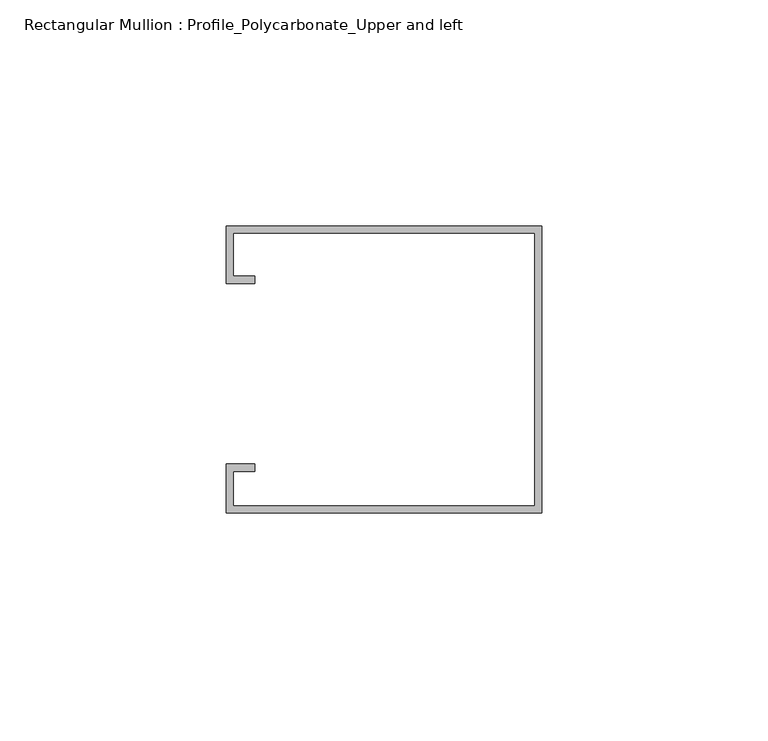
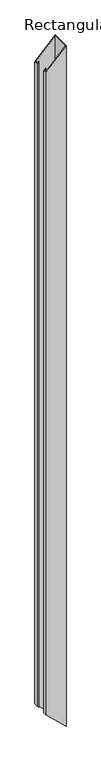
"""IFC4 building model written with IfcOpenShell, lengths in millimetres: member geometry, Rectangular Mullion : Profile_Polycarbonate_Upper and left."""

from ifc_helpers import new_model, si_unit, origin, place, context, project, spatial, faceted_brep, source, transform, mapped, element, save


def rectangular_mullion_profile_polycarbonate_upper_and_left_52db3f33(model_context):
    return source(origin(), model_context, "Body", "Brep", [
        faceted_brep([(-69.85, 32.7, -72.8210241), (0.0, 32.7, 0.0), (0.0, 32.7, -2459.5822781), (-69.85, 32.7, -2392.5820873), (-69.85, 20.0, -72.8210241), (-69.85, 20.0, -2392.5820873), (-63.5, 20.0, -66.200931), (-63.5, 20.0, -2398.6730138), (-63.5, 21.5875, -66.200931), (-63.5, 21.5875, -2398.6730138), (-68.2625, 21.5875, -71.1660008), (-68.2625, 21.5875, -2394.1048189), (-68.2625, 31.1125, -71.1660008), (-68.2625, 31.1125, -2394.1048189), (-1.5875, 31.1125, -1.6550233), (-1.5875, 31.1125, -2458.0595465), (-1.5875, -29.2125, -1.6550233), (-1.5875, -29.2125, -2458.0595465), (-68.2625, -29.2125, -71.1660008), (-68.2625, -29.2125, -2394.1048189), (-68.2625, -21.5875, -71.1660008), (-68.2625, -21.5875, -2394.1048189), (-63.5, -21.5875, -66.200931), (-63.5, -21.5875, -2398.6730138), (-63.5, -20.0, -66.200931), (-63.5, -20.0, -2398.6730138), (-69.85, -20.0, -72.8210241), (-69.85, -20.0, -2392.5820873), (-69.85, -30.8, -72.8210241), (-69.85, -30.8, -2392.5820873), (0.0, -30.8, 0.0), (0.0, -30.8, -2459.5822781)], [[[0, 1, 2, 3]], [[4, 0, 3, 5]], [[6, 4, 5, 7]], [[8, 6, 7, 9]], [[10, 8, 9, 11]], [[12, 10, 11, 13]], [[14, 12, 13, 15]], [[16, 14, 15, 17]], [[18, 16, 17, 19]], [[20, 18, 19, 21]], [[22, 20, 21, 23]], [[24, 22, 23, 25]], [[26, 24, 25, 27]], [[28, 26, 27, 29]], [[30, 28, 29, 31]], [[1, 30, 31, 2]], [[1, 0, 4, 6, 8, 10, 12, 14, 16, 18, 20, 22, 24, 26, 28, 30]], [[2, 31, 29, 27, 25, 23, 21, 19, 17, 15, 13, 11, 9, 7, 5, 3]]]),
    ])


if __name__ == "__main__":
    model = new_model("IFC4")
    model_context = context("Model", 3, world=origin())
    ifc_project = project(units=[si_unit("LENGTHUNIT", "METRE", prefix="MILLI")], contexts=[model_context])
    site = spatial("IfcSite", under=ifc_project)
    building = spatial("IfcBuilding", under=site)
    placement = place(None, origin())
    rectangular_mullion_profile_polycarbonate_upper_and_left_shape = rectangular_mullion_profile_polycarbonate_upper_and_left_52db3f33(model_context)
    element("IfcMember", 1, ObjectType="Rectangular Mullion : Profile_Polycarbonate_Upper and left", at=placement, inside=building, context=model_context, shape_type="MappedRepresentation", body=[
        mapped(rectangular_mullion_profile_polycarbonate_upper_and_left_shape, transform((0.0, 0.0, 0.0), x_axis=(1.0, 0.0, 0.0), y_axis=(0.0, 1.0, 0.0), z_axis=(0.0, 0.0, 1.0))),
    ])
    save(model, "model.ifc")

# Revit data of these elements
# Type "Rectangular Mullion : Profile_Polycarbonate_Upper and left"
#   built-in parameter 1007322 = 0.208333 (stored number, unit not read)
#   built-in parameter 1007321 = 0.00520833 (stored number, unit not read)
#   built-in parameter 1007320 = 0 (stored number, unit not read)
